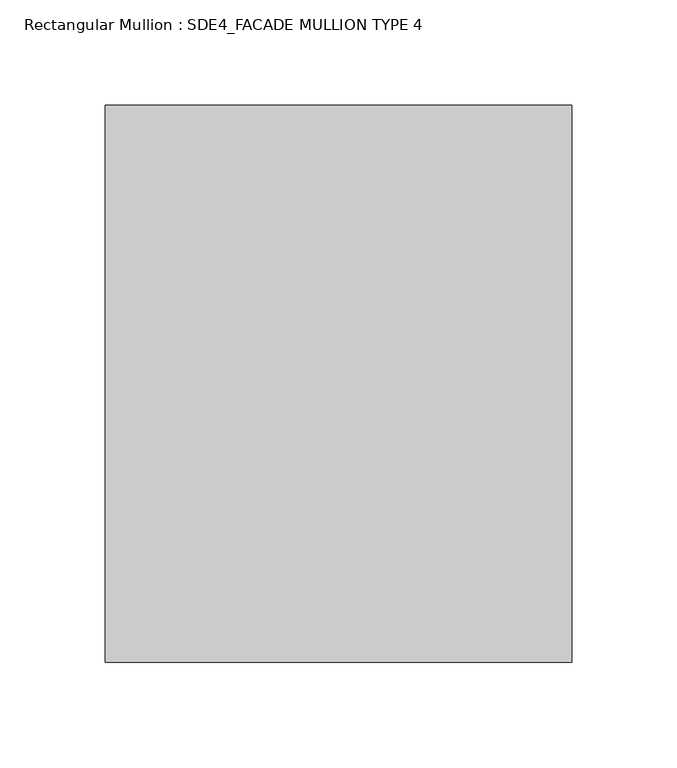
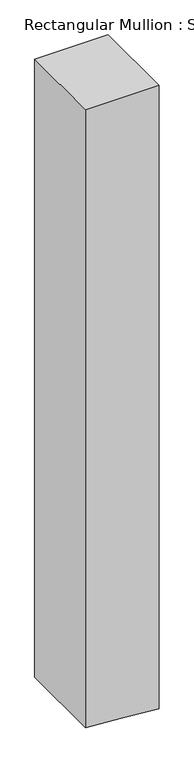
"""IFC4 building model written with IfcOpenShell, lengths in millimetres: member geometry, Rectangular Mullion : SDE4_FACADE MULLION TYPE 4."""

from ifc_helpers import new_model, si_unit, frame, origin, place, context, project, spatial, polyline, outline, extrude, source, transform, mapped, element, save


def rectangular_mullion_sde4_facade_mullion_type_4_a90e2c18(model_context):
    return source(origin(), model_context, "Body", "SweptSolid", [
        extrude(outline(polyline([(0.0, 111.0), (0.0, -111.0), (-1973.1899909, -111.0), (-1981.9309125, 3.056508), (-1990.2033524, 111.0), (0.0, 111.0)])), frame((0.0, -132.5, 0.0), z_axis=(0.0, 1.0, 0.0), x_axis=(0.0, 0.0, 1.0)), (0.0, 0.0, 1.0), 265.0),
    ])


if __name__ == "__main__":
    model = new_model("IFC4")
    model_context = context("Model", 3, world=origin())
    ifc_project = project(units=[si_unit("LENGTHUNIT", "METRE", prefix="MILLI")], contexts=[model_context])
    site = spatial("IfcSite", under=ifc_project)
    building = spatial("IfcBuilding", under=site)
    placement = place(None, origin())
    rectangular_mullion_sde4_facade_mullion_type_4_shape = rectangular_mullion_sde4_facade_mullion_type_4_a90e2c18(model_context)
    element("IfcMember", 1, ObjectType="Rectangular Mullion : SDE4_FACADE MULLION TYPE 4", at=placement, inside=building, context=model_context, shape_type="MappedRepresentation", body=[
        mapped(rectangular_mullion_sde4_facade_mullion_type_4_shape, transform((0.0, 0.0, 0.0), x_axis=(1.0, 0.0, 0.0), y_axis=(0.0, 1.0, 0.0), z_axis=(0.0, 0.0, 1.0))),
    ])
    save(model, "model.ifc")

# Revit data of these elements
# Type "Rectangular Mullion : SDE4_FACADE MULLION TYPE 4"
#   built-in parameter 1007322 = 0.869423 (stored number, unit not read)
#   built-in parameter 1007321 = 0.364173 (stored number, unit not read)
#   built-in parameter 1007320 = 0.364173 (stored number, unit not read)
